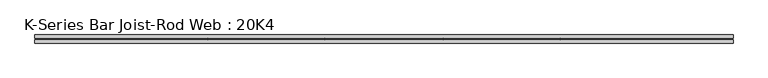
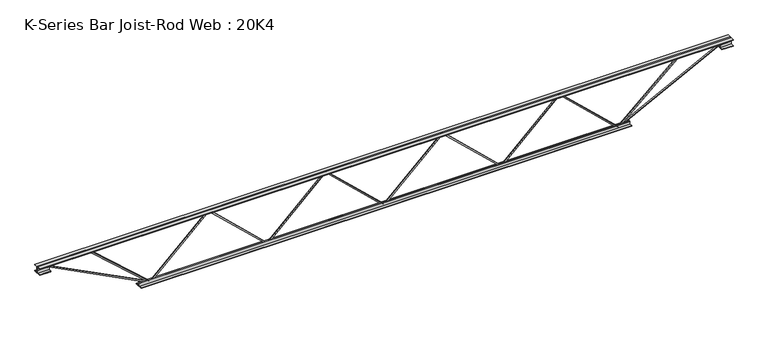
"""IFC4 building model written with IfcOpenShell, lengths in millimetres: beam geometry, K-Series Bar Joist-Rod Web : 20K4."""

from ifc_helpers import new_model, si_unit, frame, origin, place, context, project, spatial, polyline, outline, extrude, source, transform, mapped, element, save


def k_series_bar_joist_rod_web_20k4_0a7fc480(model_context):
    return source(origin(), model_context, "Body", "SweptSolid", [
        extrude(outline(polyline([(-242.8875, 0.0), (-252.4125, 0.0), (-252.4125, 5.0783169), (242.8875, 525.7783169), (242.8875, 528.3216831), (-252.4125, 1049.0216831), (-252.4125, 1054.1), (-242.8875, 1054.1), (-242.8875, 1052.8283169), (252.4125, 532.1283169), (252.4125, 521.9716831), (-242.8875, 1.2716831), (-242.8875, 0.0)])), frame((0.0, -4.7625, 0.0), z_axis=(0.0, 1.0, 0.0), x_axis=(0.0, 0.0, 1.0)), (0.0, 0.0, 1.0), 9.525),
        extrude(outline(polyline([(-242.8875, -1054.1), (-252.4125, -1054.1), (-252.4125, -1049.0216831), (242.8875, -528.3216831), (242.8875, -525.7783169), (-252.4125, -5.0783169), (-252.4125, 0.0), (-242.8875, 0.0), (-242.8875, -1.2716831), (252.4125, -521.9716831), (252.4125, -532.1283169), (-242.8875, -1052.8283169), (-242.8875, -1054.1)])), frame((0.0, -4.7625, 0.0), z_axis=(0.0, 1.0, 0.0), x_axis=(0.0, 0.0, 1.0)), (0.0, 0.0, 1.0), 9.525),
        extrude(outline(polyline([(-242.8875, 1054.1), (-252.4125, 1054.1), (-252.4125, 1059.1783169), (242.8875, 1579.8783169), (242.8875, 1582.4216831), (-252.4125, 2103.1216831), (-252.4125, 2108.2), (-242.8875, 2108.2), (-242.8875, 2106.9283169), (252.4125, 1586.2283169), (252.4125, 1576.0716831), (-242.8875, 1055.3716831), (-242.8875, 1054.1)])), frame((0.0, -4.7625, 0.0), z_axis=(0.0, 1.0, 0.0), x_axis=(0.0, 0.0, 1.0)), (0.0, 0.0, 1.0), 9.525),
        extrude(outline(polyline([(-242.8875, -2108.2), (-252.4125, -2108.2), (-252.4125, -2103.1216831), (242.8875, -1582.4216831), (242.8875, -1579.8783169), (-252.4125, -1059.1783169), (-252.4125, -1054.1), (-242.8875, -1054.1), (-242.8875, -1055.3716831), (252.4125, -1576.0716831), (252.4125, -1586.2283169), (-242.8875, -2106.9283169), (-242.8875, -2108.2)])), frame((0.0, -4.7625, 0.0), z_axis=(0.0, 1.0, 0.0), x_axis=(0.0, 0.0, 1.0)), (0.0, 0.0, 1.0), 9.525),
        extrude(outline(polyline([(4.7625, 254.0), (36.5125, 254.0), (36.5125, 247.65), (11.1125, 247.65), (11.1125, 222.25), (4.7625, 222.25), (4.7625, 254.0)])), frame((-3124.2, 0.0, 0.0), z_axis=(1.0, 0.0, 0.0), x_axis=(0.0, 1.0, 0.0)), (0.0, 0.0, 1.0), 6248.4),
        extrude(outline(polyline([(-4.7625, 254.0), (-4.7625, 222.25), (-11.1125, 222.25), (-11.1125, 247.65), (-36.5125, 247.65), (-36.5125, 254.0), (-4.7625, 254.0)])), frame((-3124.2, 0.0, 0.0), z_axis=(1.0, 0.0, 0.0), x_axis=(0.0, 1.0, 0.0)), (0.0, 0.0, 1.0), 6248.4),
        extrude(outline(polyline([(-4.7625, 190.5), (-36.5125, 190.5), (-36.5125, 196.85), (-11.1125, 196.85), (-11.1125, 222.25), (-4.7625, 222.25), (-4.7625, 190.5)])), frame((-3124.2, 0.0, 0.0), z_axis=(1.0, 0.0, 0.0), x_axis=(0.0, 1.0, 0.0)), (0.0, 0.0, 1.0), 101.6),
        extrude(outline(polyline([(36.5125, 190.5), (4.7625, 190.5), (4.7625, 222.25), (11.1125, 222.25), (11.1125, 196.85), (36.5125, 196.85), (36.5125, 190.5)])), frame((-3124.2, 0.0, 0.0), z_axis=(1.0, 0.0, 0.0), x_axis=(0.0, 1.0, 0.0)), (0.0, 0.0, 1.0), 101.6),
        extrude(outline(polyline([(4.7625, 190.5), (4.7625, 222.25), (11.1125, 222.25), (11.1125, 196.85), (36.5125, 196.85), (36.5125, 190.5), (4.7625, 190.5)])), frame((3022.6, 0.0, 0.0), z_axis=(1.0, 0.0, 0.0), x_axis=(0.0, 1.0, 0.0)), (0.0, 0.0, 1.0), 101.6),
        extrude(outline(polyline([(-4.7625, 190.5), (-36.5125, 190.5), (-36.5125, 196.85), (-11.1125, 196.85), (-11.1125, 222.25), (-4.7625, 222.25), (-4.7625, 190.5)])), frame((3022.6, 0.0, 0.0), z_axis=(1.0, 0.0, 0.0), x_axis=(0.0, 1.0, 0.0)), (0.0, 0.0, 1.0), 101.6),
        extrude(outline(polyline([(4.7625, -254.0), (4.7625, -222.25), (11.1125, -222.25), (11.1125, -247.65), (36.5125, -247.65), (36.5125, -254.0), (4.7625, -254.0)])), frame((-2209.8, 0.0, 0.0), z_axis=(1.0, 0.0, 0.0), x_axis=(0.0, 1.0, 0.0)), (0.0, 0.0, 1.0), 4419.6),
        extrude(outline(polyline([(-4.7625, -254.0), (-36.5125, -254.0), (-36.5125, -247.65), (-11.1125, -247.65), (-11.1125, -222.25), (-4.7625, -222.25), (-4.7625, -254.0)])), frame((-2209.8, 0.0, 0.0), z_axis=(1.0, 0.0, 0.0), x_axis=(0.0, 1.0, 0.0)), (0.0, 0.0, 1.0), 4419.6),
        extrude(outline(polyline([(0.0, -9.525), (0.0, 0.0), (1028.0726482, 0.0), (1028.0726482, -9.525), (0.0, -9.525)])), frame((-3024.7767905, 4.7625, 218.0140834), z_axis=(0.45706886650213835, 0.0, 0.8894313077885501), x_axis=(0.8894313077885501, 0.0, -0.45706886650213835)), (0.0, 0.0, 1.0), 9.525),
        extrude(outline(polyline([(0.0, -9.525), (0.0, 0.0), (706.1074369, 0.0), (706.1074369, -9.525), (0.0, -9.525)])), frame((-2638.419346, 4.7625, 218.695193), z_axis=(0.6654794658970488, 0.0, 0.7464161576958116), x_axis=(0.7464161576958116, 0.0, -0.6654794658970488)), (0.0, 0.0, 1.0), 9.525),
        extrude(outline(polyline([(0.0, -9.525), (0.0, 0.0), (1028.0726482, 0.0), (1028.0726482, -9.525), (0.0, -9.525)])), frame((3024.7767905, -4.7625, 218.0140834), z_axis=(-0.4570688665021271, 0.0, 0.8894313077885558), x_axis=(-0.8894313077885558, 0.0, -0.4570688665021271)), (0.0, 0.0, 1.0), 9.525),
        extrude(outline(polyline([(0.0, -9.525), (0.0, 0.0), (706.1074369, 0.0), (706.1074369, -9.525), (0.0, -9.525)])), frame((2638.419346, -4.7625, 218.695193), z_axis=(-0.6654794658970452, 0.0, 0.7464161576958149), x_axis=(-0.7464161576958149, 0.0, -0.6654794658970452)), (0.0, 0.0, 1.0), 9.525),
    ])


if __name__ == "__main__":
    model = new_model("IFC4")
    model_context = context("Model", 3, world=origin())
    ifc_project = project(units=[si_unit("LENGTHUNIT", "METRE", prefix="MILLI")], contexts=[model_context])
    site = spatial("IfcSite", under=ifc_project)
    building = spatial("IfcBuilding", under=site)
    placement = place(None, origin())
    k_series_bar_joist_rod_web_20k4_shape = k_series_bar_joist_rod_web_20k4_0a7fc480(model_context)
    element("IfcBeam", 1, ObjectType="K-Series Bar Joist-Rod Web : 20K4", at=placement, inside=building, context=model_context, shape_type="MappedRepresentation", body=[
        mapped(k_series_bar_joist_rod_web_20k4_shape, transform((0.0, 0.0, 0.0), x_axis=(1.0, 0.0, 0.0), y_axis=(0.0, 1.0, 0.0), z_axis=(0.0, 0.0, 1.0))),
    ])
    save(model, "model.ifc")

# Revit data of these elements
# Type "K-Series Bar Joist-Rod Web : 20K4"
#   Assembly Code = "B1010350"
#   Wt = 7.6
#   Web Thickness = 0' - 0 3/8"
#   Start Offset [instance default] = 0' - 0"
#   Start Extension [instance default] = 0' - 0"
#   Seat Length = 0' - 4"
#   Seat Depth = 0' - 2 1/2"
#   PanelArrayLength [instance default] = 17' - 4"
#   Panel [instance default] = 3' - 5.6"
#   End Offset [instance default] = 0' - 0"
#   End Extension [instance default] = 0' - 0"
#   End Panel = 3' - 4"
#   Cord Leg = 0' - 1 1/4"
#   Chord Thickness = 0' - 0 1/4"
#   Length [instance default] = 24' - 0"
#   Depth = 1' - 8"
#   PanelArrayNum [instance default] = 5
#   Structural Material = none
# Element 1 (IfcBeam, "K-Series Bar Joist-Rod Web : 20K4")
#   PanelArrayLength = 13' - 10"
#   Panel = 3' - 5 1/2"
#   PanelArrayNum = 4
